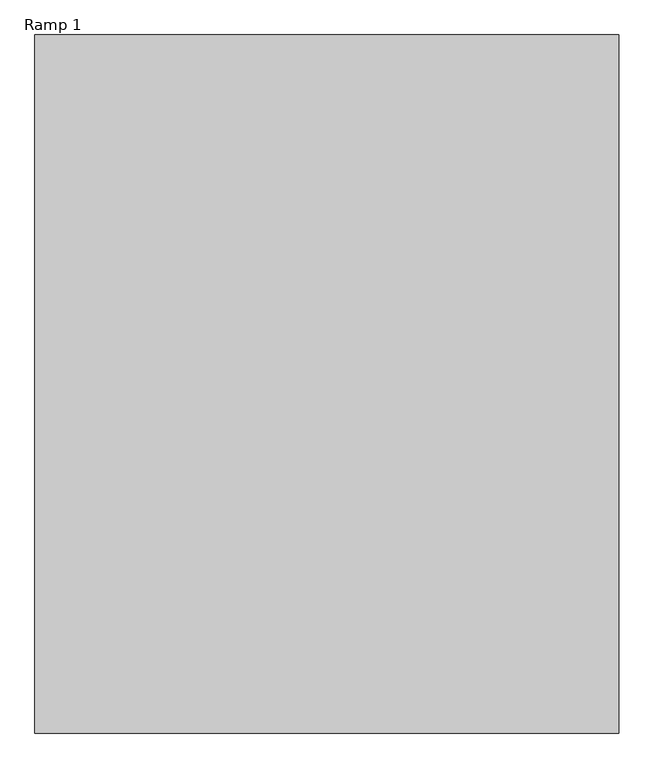
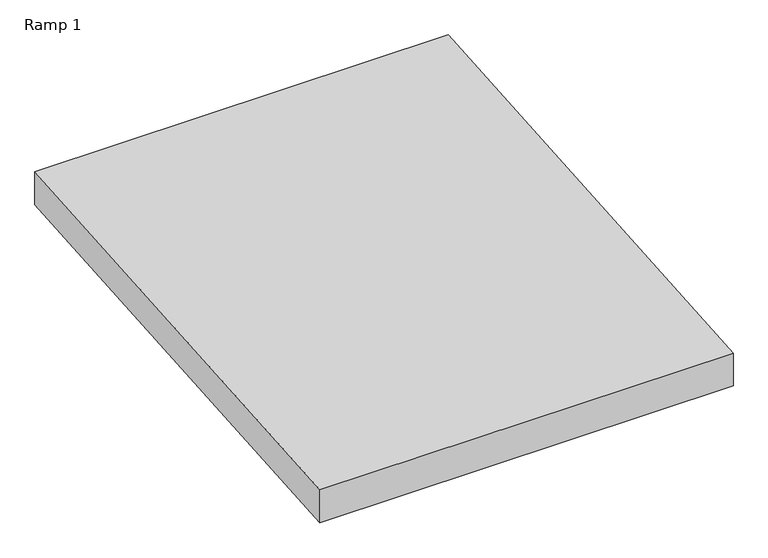
"""IFC4 building model written with IfcOpenShell, lengths in millimetres: ramp geometry, Ramp 1."""

from ifc_helpers import new_model, si_unit, frame, origin, place, context, project, spatial, polyline, outline, extrude, source, transform, mapped, element, save


def ramp_1_b614bedc(model_context):
    return source(origin(), model_context, "Body", "SweptSolid", [
        extrude(outline(polyline([(-588.7354398, 40.0), (1550.939444, 200.0), (1550.939444, 49.5812066), (-588.7354398, -110.4187934), (-588.7354398, 40.0)])), frame((5737.3508412, 0.0, 0.0), z_axis=(1.0, 0.0, 0.0), x_axis=(0.0, 1.0, 0.0)), (0.0, 0.0, 1.0), 1790.0),
    ])


if __name__ == "__main__":
    model = new_model("IFC4")
    model_context = context("Model", 3, world=origin())
    ifc_project = project(units=[si_unit("LENGTHUNIT", "METRE", prefix="MILLI")], contexts=[model_context])
    site = spatial("IfcSite", under=ifc_project)
    building = spatial("IfcBuilding", under=site)
    placement = place(None, origin())
    ramp_1_shape = ramp_1_b614bedc(model_context)
    element("IfcRamp", 1, ObjectType="Ramp 1", at=placement, inside=building, context=model_context, shape_type="MappedRepresentation", body=[
        mapped(ramp_1_shape, transform((0.0, 0.0, 0.0), x_axis=(1.0, 0.0, 0.0), y_axis=(0.0, 1.0, 0.0), z_axis=(0.0, 0.0, 1.0))),
    ])
    save(model, "model.ifc")
